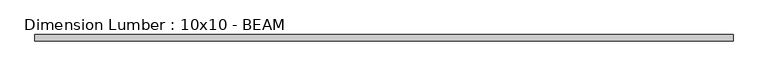
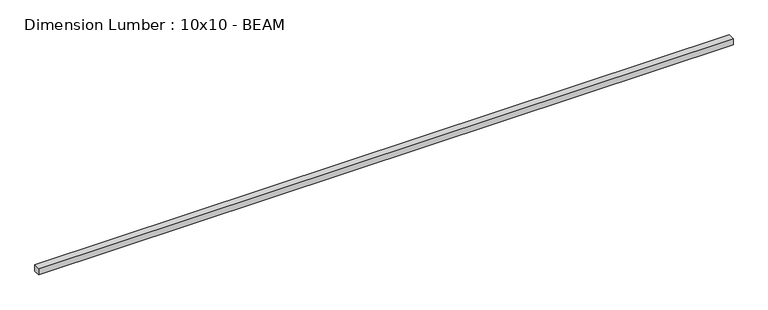
"""IFC4 building model written with IfcOpenShell, lengths in millimetres: beam geometry, Dimension Lumber : 10x10 - BEAM."""

from ifc_helpers import new_model, si_unit, frame, origin, place, context, project, spatial, polyline, outline, extrude, source, transform, mapped, element, save


def dimension_lumber_10x10_beam_db3298f4(model_context):
    return source(origin(), model_context, "Body", "SweptSolid", [
        extrude(outline(polyline([(12496.8, 117.475), (12496.8, -117.475), (-12496.8, -117.475), (-12496.8, 117.475), (12496.8, 117.475)])), frame((0.0, 0.0, -117.475), z_axis=(0.0, 0.0, 1.0), x_axis=(1.0, 0.0, 0.0)), (0.0, 0.0, 1.0), 234.95),
    ])


if __name__ == "__main__":
    model = new_model("IFC4")
    model_context = context("Model", 3, world=origin())
    ifc_project = project(units=[si_unit("LENGTHUNIT", "METRE", prefix="MILLI")], contexts=[model_context])
    site = spatial("IfcSite", under=ifc_project)
    building = spatial("IfcBuilding", under=site)
    placement = place(None, origin())
    dimension_lumber_10x10_beam_shape = dimension_lumber_10x10_beam_db3298f4(model_context)
    element("IfcBeam", 1, ObjectType="Dimension Lumber : 10x10 - BEAM", at=placement, inside=building, context=model_context, shape_type="MappedRepresentation", body=[
        mapped(dimension_lumber_10x10_beam_shape, transform((0.0, 0.0, 0.0), x_axis=(1.0, 0.0, 0.0), y_axis=(0.0, 1.0, 0.0), z_axis=(0.0, 0.0, 1.0))),
    ])
    save(model, "model.ifc")

# Revit data of these elements
# Type "Dimension Lumber : 10x10 - BEAM"
#   Assembly Code = "B10"
#   A = 0.0755556 SF
#   Length [instance default] = 5' - 0"
#   b = 0' - 9 1/4"
#   d = 0' - 9 1/4"
#   Structural Material = (4) CHARRED SISTERED 2X10s AT BEAM
# Element 1 (IfcBeam, "Dimension Lumber : 10x10 - BEAM")
#   Materials on its faces: "(4) CHARRED SISTERED 2X10s AT BEAM"
# Materials
#   "(4) CHARRED SISTERED 2X10s AT BEAM": class "Wood", colour RGB 144 144 144, transparency 0, Description = "Pinus Echinata", Cost = 0
